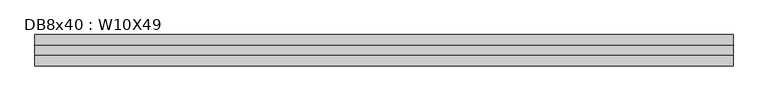
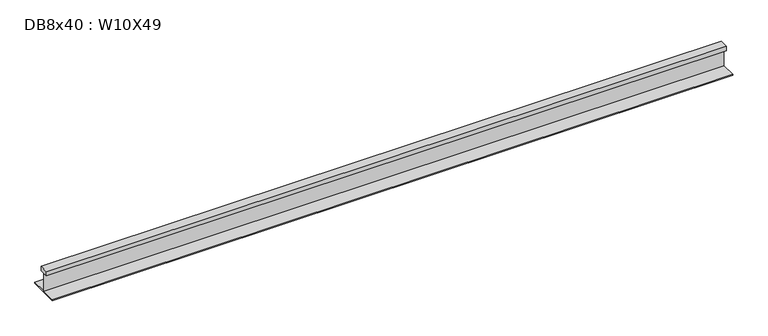
"""IFC4 building model written with IfcOpenShell, lengths in millimetres: beam geometry, DB8x40 : W10X49."""

from ifc_helpers import new_model, si_unit, frame, origin, place, context, project, spatial, polyline, outline, extrude, source, transform, mapped, element, save


def db8x40_w10x49_5f415a01(model_context):
    return source(origin(), model_context, "Body", "SweptSolid", [
        extrude(outline(polyline([(38.1, 144.3355), (38.1, 106.2355), (2.921, 106.2355), (2.921, -49.53), (127.0, -49.53), (127.0, -59.182), (-127.0, -59.182), (-127.0, -49.53), (-2.921, -49.53), (-2.921, 106.2355), (-38.1, 106.2355), (-38.1, 144.3355), (38.1, 144.3355)])), frame((-2911.6465755, 0.0, 0.0), z_axis=(1.0, 0.0, 0.0), x_axis=(0.0, 1.0, 0.0)), (0.0, 0.0, 1.0), 5675.0595426),
    ])


if __name__ == "__main__":
    model = new_model("IFC4")
    model_context = context("Model", 3, world=origin())
    ifc_project = project(units=[si_unit("LENGTHUNIT", "METRE", prefix="MILLI")], contexts=[model_context])
    site = spatial("IfcSite", under=ifc_project)
    building = spatial("IfcBuilding", under=site)
    placement = place(None, origin())
    db8x40_w10x49_shape = db8x40_w10x49_5f415a01(model_context)
    element("IfcBeam", 1, ObjectType="DB8x40 : W10X49", at=placement, inside=building, context=model_context, shape_type="MappedRepresentation", body=[
        mapped(db8x40_w10x49_shape, transform((0.0, 0.0, 0.0), x_axis=(1.0, 0.0, 0.0), y_axis=(0.0, 1.0, 0.0), z_axis=(0.0, 0.0, 1.0))),
    ])
    save(model, "model.ifc")

# Revit data of these elements
# Type "DB8x40 : W10X49"
#   Assembly Code = "B10"
#   W = 53
#   Length [instance default] = 5' - 0"
#   bf = 0' - 10"
#   d = 1' - 0.1"
#   k = 0' - 1 3/8"
#   k2 = 0' - 0.8"
#   tf = 0' - 0.575"
#   tw = 0' - 0.345"
#   A = 0.108333 SF
#   Structural Material [instance default] = Steel ASTM A992
# Element 1 (IfcBeam, "DB8x40 : W10X49")
#   Materials on its faces: "Steel ASTM A992"
# Materials
#   "Steel ASTM A992": class "Metal", colour RGB 199 199 199, transparency 0, Description = "Structural steel 50ksi", Cost = 0
